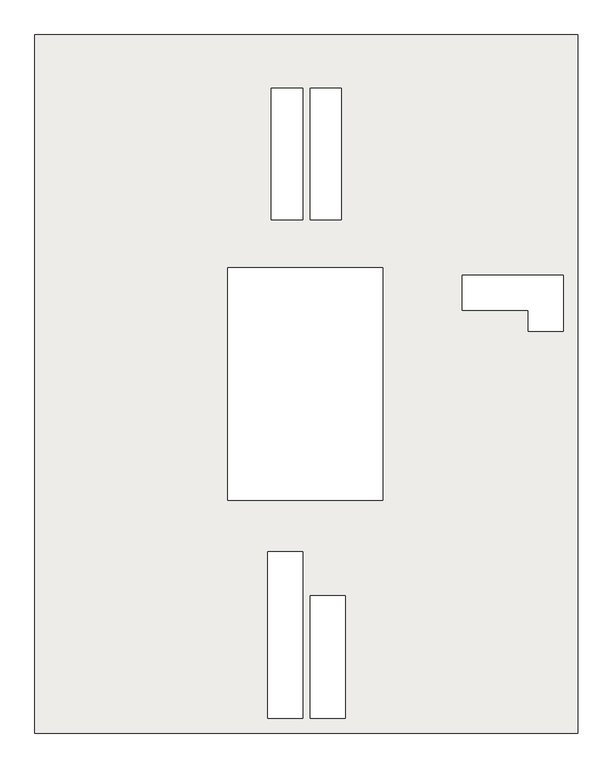
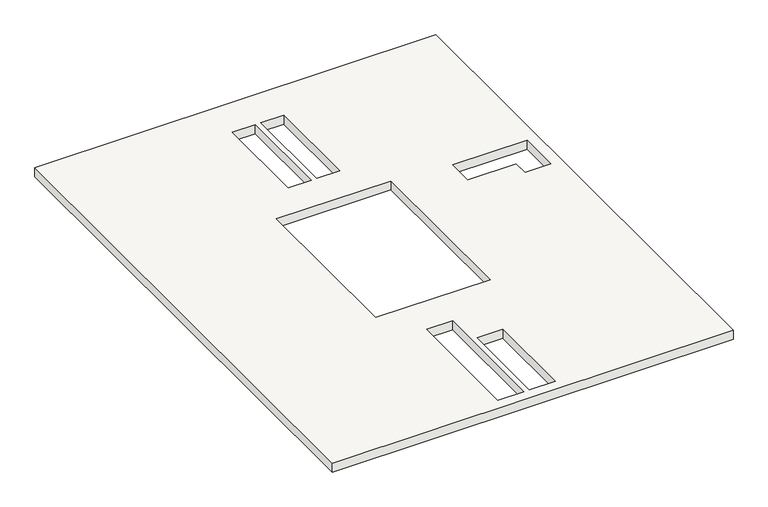
"""IFC4 building model written with IfcOpenShell, lengths in millimetres: slab geometry, Holzdecke 142136 : Holzdecke 142136."""

from ifc_helpers import new_model, si_unit, frame, origin, place, context, project, spatial, polyline, outline, extrude, source, transform, mapped, element, save


def slab_52cff1b9(model_context):
    return source(origin(), model_context, "Body", "SweptSolid", [
        extrude(outline(polyline([(172797.7593015, 28481.9343946), (158797.7593015, 28481.9343946), (158797.7593015, 46484.7962965), (172797.7593015, 46484.7962965), (172797.7593015, 28481.9343946)]), holes=[polyline([(167772.7593015, 40484.7962965), (163772.7593015, 40484.7962965), (163772.7593015, 34484.7962965), (167772.7593015, 34484.7962965), (167772.7593015, 40484.7962965)]), polyline([(165697.7593015, 33159.7962965), (164797.7593015, 33159.7962965), (164797.7593015, 28861.9343946), (165697.7593015, 28861.9343946), (165697.7593015, 33159.7962965)]), polyline([(165897.7593015, 32021.9343946), (165897.7593015, 29779.7962965), (165897.7593015, 28861.9343946), (166797.7593015, 28861.9343946), (166797.7593015, 32021.9343946), (165897.7593015, 32021.9343946)]), polyline([(171517.7593015, 38844.7962965), (172417.7593015, 38844.7962965), (172417.7593015, 40284.7962965), (169822.7593015, 40284.7962965), (169822.7593015, 39384.7962965), (171517.7593015, 39384.7962965), (171517.7593015, 38844.7962965)]), polyline([(165897.7593015, 45104.7962965), (165897.7593015, 41724.7962965), (166697.7593015, 41724.7962965), (166697.7593015, 45104.7962965), (165897.7593015, 45104.7962965)]), polyline([(164897.7593015, 41724.7962965), (165697.7593015, 41724.7962965), (165697.7593015, 45104.7962965), (164897.7593015, 45104.7962965), (164897.7593015, 41724.7962965)])]), frame((0.0, 0.0, 5830.0), z_axis=(0.0, 0.0, 1.0), x_axis=(1.0, 0.0, 0.0)), (0.0, 0.0, 1.0), 330.0),
    ])


if __name__ == "__main__":
    model = new_model("IFC4")
    model_context = context("Model", 3, world=origin())
    ifc_project = project(units=[si_unit("LENGTHUNIT", "METRE", prefix="MILLI")], contexts=[model_context])
    site = spatial("IfcSite", under=ifc_project)
    building = spatial("IfcBuilding", under=site)
    placement = place(None, origin())
    slab_shape = slab_52cff1b9(model_context)
    element("IfcSlab", 1, ObjectType="Holzdecke 142136 : Holzdecke 142136", at=placement, inside=building, context=model_context, shape_type="MappedRepresentation", body=[
        mapped(slab_shape, transform((0.0, 0.0, 0.0), x_axis=(1.0, 0.0, 0.0), y_axis=(0.0, 1.0, 0.0), z_axis=(0.0, 0.0, 1.0))),
    ])
    save(model, "model.ifc")

# Revit data of these elements
# Type "Holzdecke 142136 : Holzdecke 142136"
#   Abrechnungsart = "m²"
#   Allright_Bauteil_ID = "0123De 0783954319"
#   Bezeichnung = "Holzdecke"
#   Codetext = "D-HOLZBALKEN1\\"
#   Gewerk = "Zimmer- und Holzbauarbeiten"
#   Material = "Holz"
#   Objektname = "Brettstapeldecke"
#   NameOverride = "Holzdecke"
#   Reference = "Holzdecke"
#   Status = "NEW"
#   PitchAngle = 0.00°
#   ThermalTransmittance = 0.0000 BTU/(h·ft²·°F)
#   2D Interaktion = yes
#   Combustible = no
#   Compartmentation = no
#   IsExternal = no
#   LoadBearing = yes
# Element 1 (IfcSlab, "Holzdecke 142136 : Holzdecke 142136")
#   Materials on its faces: "holzschalung"
# Materials
#   "holzschalung": class "Unassigned", colour RGB 128 128 128, transparency 0
